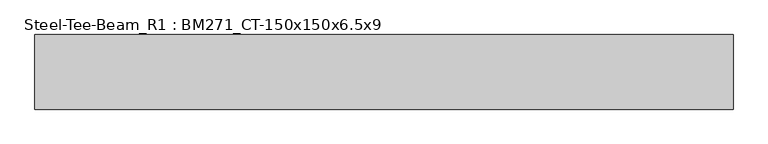
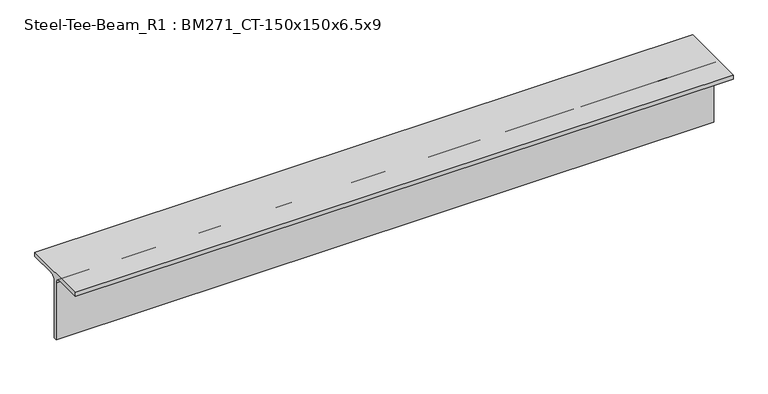
"""IFC4 building model written with IfcOpenShell, lengths in millimetres: member geometry, Steel-Tee-Beam_R1 : BM271_CT-150x150x6.5x9."""

from ifc_helpers import new_model, si_unit, point, frame, frame_2d, origin, place, context, project, spatial, polyline, circle_curve, trimmed, segment, composite_curve, outline, extrude, source, transform, mapped, element, save


def steel_tee_beam_r1_bm271_ct_150x150x6_5x9_5363d751(model_context):
    return source(origin(), model_context, "Body", "SweptSolid", [
        extrude(outline(composite_curve([segment(polyline([(-75.0, 75.0), (75.0, 75.0), (75.0, 66.0), (16.25, 66.0)]), True, "CONTINUOUS"), segment(trimmed(circle_curve(frame_2d((16.25, 53.0)), 13.0), [point((16.25, 66.0))], [point((3.25, 53.0))], True, "CARTESIAN"), True, "CONTINUOUS"), segment(polyline([(3.25, 53.0), (3.25, -75.0), (-3.25, -75.0), (-3.25, 53.0)]), True, "CONTINUOUS"), segment(trimmed(circle_curve(frame_2d((-16.25, 53.0)), 13.0), [point((-3.25, 53.0))], [point((-16.25, 66.0))], True, "CARTESIAN"), True, "CONTINUOUS"), segment(polyline([(-16.25, 66.0), (-75.0, 66.0), (-75.0, 75.0)]), True, "CONTINUOUS")], self_intersect=False)), frame((-701.7933274, 0.0, 0.0), z_axis=(1.0, 0.0, 0.0), x_axis=(0.0, 1.0, 0.0)), (0.0, 0.0, 1.0), 1403.5866548),
    ])


if __name__ == "__main__":
    model = new_model("IFC4")
    model_context = context("Model", 3, world=origin())
    ifc_project = project(units=[si_unit("LENGTHUNIT", "METRE", prefix="MILLI")], contexts=[model_context])
    site = spatial("IfcSite", under=ifc_project)
    building = spatial("IfcBuilding", under=site)
    placement = place(None, origin())
    steel_tee_beam_r1_bm271_ct_150x150x6_5x9_shape = steel_tee_beam_r1_bm271_ct_150x150x6_5x9_5363d751(model_context)
    element("IfcMember", 1, ObjectType="Steel-Tee-Beam_R1 : BM271_CT-150x150x6.5x9", at=placement, inside=building, context=model_context, shape_type="MappedRepresentation", body=[
        mapped(steel_tee_beam_r1_bm271_ct_150x150x6_5x9_shape, transform((0.0, 0.0, 0.0), x_axis=(1.0, 0.0, 0.0), y_axis=(0.0, 1.0, 0.0), z_axis=(0.0, 0.0, 1.0))),
    ])
    save(model, "model.ifc")

# Revit data of these elements
# Type "Steel-Tee-Beam_R1 : BM271_CT-150x150x6.5x9"
#   Keynote = "CT-150x150x6.5x9"
#   Surface Area = 0.588841 m²/m
#   Section Area = 23.3904 cm²
#   Mass per Unit Length = 18.3614 kg/m
#   Length [instance default] = 1.5240 m
#   bf = 0.1500 m
#   d = 0.1500 m
#   k = 0.0220 m
#   r = 0.0130 m
#   tf = 0.0090 m
#   tw = 0.0065 m
#   hec_material4 [instance default] = none
#   hec_material3 [instance default] = none
#   hec_material2 [instance default] = none
#   hec_material1 [instance default] = none
#   Structural Material [instance default] = Steel, 45-345
#   Assembly Code = ""
# Element 1 (IfcMember, "Steel-Tee-Beam_R1 : BM271_CT-150x150x6.5x9")
#   Structural Material = none
# Materials
#   "Steel, 45-345": class "Metal", colour RGB 189 187 185, transparency 0, Description = "Steel 345 MPa", Cost = 0
